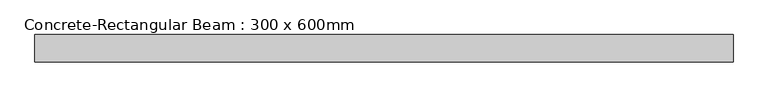
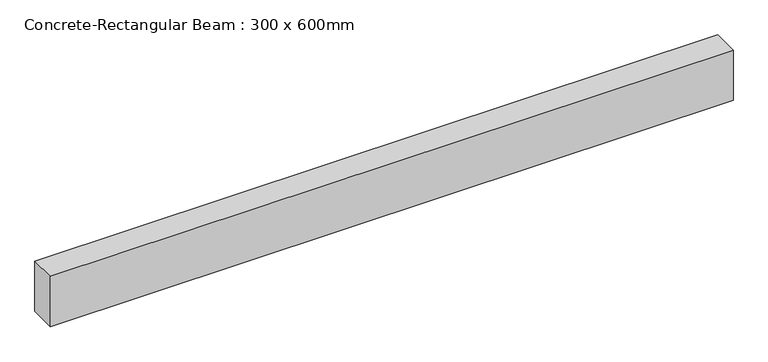
"""IFC4 building model written with IfcOpenShell, lengths in millimetres: beam geometry, Concrete-Rectangular Beam : 300 x 600mm."""

from ifc_helpers import new_model, si_unit, frame, origin, place, context, project, spatial, polyline, outline, extrude, source, transform, mapped, element, save


def concrete_rectangular_beam_300_x_600mm_526adf45(model_context):
    return source(origin(), model_context, "Body", "SweptSolid", [
        extrude(outline(polyline([(3850.0, 150.0), (3850.0, -150.0), (-3850.0, -150.0), (-3850.0, 150.0), (3850.0, 150.0)])), frame((0.0, 0.0, -300.0), z_axis=(0.0, 0.0, 1.0), x_axis=(1.0, 0.0, 0.0)), (0.0, 0.0, 1.0), 600.0),
    ])


if __name__ == "__main__":
    model = new_model("IFC4")
    model_context = context("Model", 3, world=origin())
    ifc_project = project(units=[si_unit("LENGTHUNIT", "METRE", prefix="MILLI")], contexts=[model_context])
    site = spatial("IfcSite", under=ifc_project)
    building = spatial("IfcBuilding", under=site)
    placement = place(None, origin())
    concrete_rectangular_beam_300_x_600mm_shape = concrete_rectangular_beam_300_x_600mm_526adf45(model_context)
    element("IfcBeam", 1, ObjectType="Concrete-Rectangular Beam : 300 x 600mm", at=placement, inside=building, context=model_context, shape_type="MappedRepresentation", body=[
        mapped(concrete_rectangular_beam_300_x_600mm_shape, transform((0.0, 0.0, 0.0), x_axis=(1.0, 0.0, 0.0), y_axis=(0.0, 1.0, 0.0), z_axis=(0.0, 0.0, 1.0))),
    ])
    save(model, "model.ifc")

# Revit data of these elements
# Type "Concrete-Rectangular Beam : 300 x 600mm"
#   Length [instance default] = 1524 mm
#   b = 300 mm
#   h = 600 mm
#   Structural Material [instance default] = Concrete, Cast-in-Place gray
#   Assembly Code = ""
# Element 1 (IfcBeam, "Concrete-Rectangular Beam : 300 x 600mm")
#   Materials on its faces: "Concrete, Cast-in-Place gray"
# Materials
#   "Concrete, Cast-in-Place gray": class "Concrete", colour RGB 192 192 192, transparency 0, Description = "Cast-in-place concrete", Cost = 0
